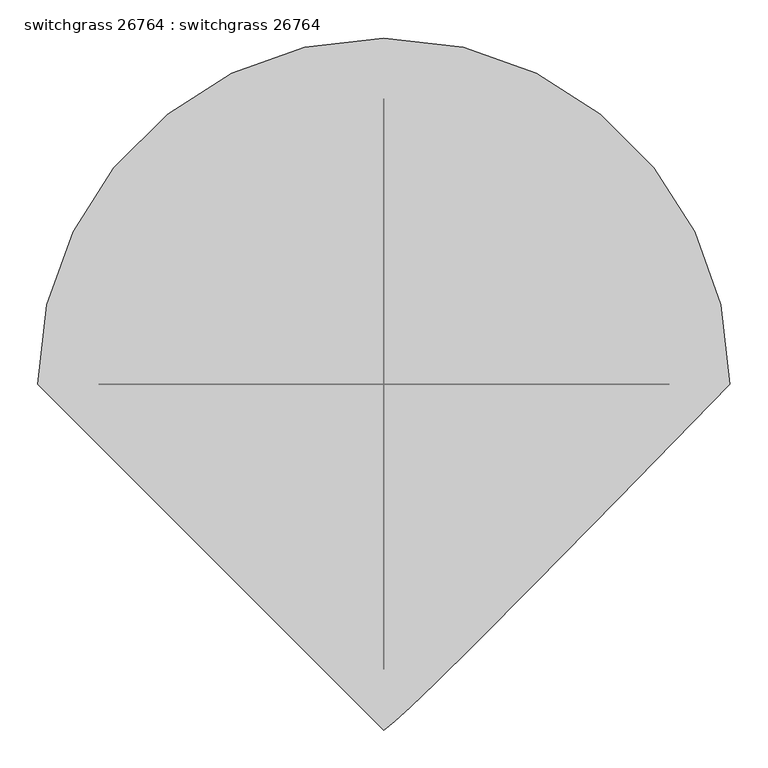
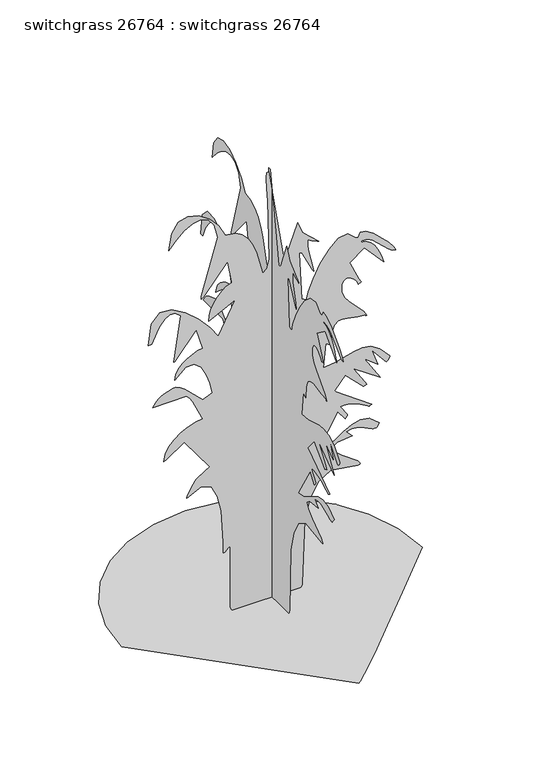
"""IFC4 building model written with IfcOpenShell, lengths in millimetres: proxy geometry, switchgrass 26764 : switchgrass 26764."""

from ifc_helpers import new_model, si_unit, origin, place, context, project, spatial, triangles, source, transform, mapped, element, save


def switchgrass_26764_switchgrass_26764_1a5b5e56(model_context):
    return source(origin(), model_context, "Body", "Tessellation", [
        triangles([(-457.5348269, 0.0, 5.72e-05), (-445.4393443, 104.8366151, 5.72e-05), (-410.9893759, 201.1121793, 5.72e-05), (-356.9483794, 286.0697479, 5.72e-05), (-286.0697479, 356.9483794, 5.72e-05), (-201.1121793, 410.9893759, 5.72e-05), (-104.8366151, 445.4393443, 5.72e-05), (2e-05, 457.5348269, 5.72e-05), (104.8366151, 445.4393443, 5.72e-05), (201.1124336, 410.9893759, 5.72e-05), (286.0697479, 356.9483794, 5.72e-05), (356.9483794, 286.0697479, 5.72e-05), (410.9893759, 201.1121793, 5.72e-05), (445.4393443, 104.8366151, 5.72e-05), (457.5348269, -4e-05, 5.72e-05), (308.8459013, -152.5179615, 5.72e-05), (198.615602, -264.8099809, 5.72e-05), (120.4339824, -343.5803727, 5.72e-05), (67.8913365, -395.5334879, 5.72e-05), (34.5780016, -427.3748946, 5.72e-05), (14.0840831, -445.8076721, 5.72e-05), (-6e-05, -457.5348269, 5.72e-05), (34.93284, -5.5e-06, 1088.4574717), (36.237382, -5.5e-06, 1088.5946726), (37.9539129, -5.5e-06, 1088.9655075), (39.8896437, -5.5e-06, 1089.5065355), (41.8515379, -5.4e-06, 1090.1567139), (43.6465546, -5.4e-06, 1090.8526743), (45.0816551, -5.3e-06, 1091.5334467), (45.9643001, -5.3e-06, 1092.1353722), (79.0584374, -3e-07, 1176.7097157), (93.7670509, -2.4e-06, 1139.9381956), (141.570056, -5.1e-06, 1095.8133453), (139.9581813, -5e-06, 1096.2705122), (120.3097713, -3.5e-06, 1104.9699812), (109.4510318, -2.7e-06, 1111.5257584), (108.7718309, -3.8e-06, 1094.9344746), (110.1157441, -4.9e-06, 1079.5497305), (124.110375, -9.5e-06, 1020.4566805), (126.8614426, -1.06e-05, 1003.8832008), (124.028585, -1.03e-05, 1007.8913137), (90.0899044, -6.2e-06, 1077.4263136), (82.7355931, -6.2e-06, 1077.4263136), (90.0899044, -1.52e-05, 926.664731), (91.5981517, -1.52e-05, 926.3243448), (93.839948, -1.52e-05, 925.4277426), (96.493992, -1.53e-05, 924.1679358), (99.2384648, -1.54e-05, 922.7353924), (101.7517925, -1.55e-05, 921.3205805), (103.7124104, -1.55e-05, 920.1165842), (104.7985178, -1.56e-05, 919.30893), (110.3578079, -1.41e-05, 944.2085003), (125.3806282, -1.19e-05, 981.1629307), (147.3843723, -9.5e-06, 1022.163553), (173.8869515, -7.3e-06, 1059.1942142), (202.4055415, -5.8e-06, 1084.2512604), (230.4577718, -5.5e-06, 1089.3210817), (255.5618354, -6.8e-06, 1066.3950829), (262.9151293, -6.8e-06, 1066.3950829), (269.3514915, -6.1e-06, 1080.2456909), (285.9199024, -6.4e-06, 1077.2713085), (308.5106383, -7.4e-06, 1062.4834757), (355.3227882, -1.03e-05, 1017.5331671), (371.3222114, -1.13e-05, 997.3934807), (376.9076989, -1.17e-05, 985.4987125), (366.3362148, -1.13e-05, 987.6501074), (353.3212752, -1.07e-05, 997.467168), (306.0061764, -8.2e-06, 1041.5234179), (289.6028898, -7.7e-06, 1050.6166128), (273.9463418, -7.7e-06, 1051.6859516), (270.2709666, -7.9e-06, 1048.0105946), (286.0621357, -8.1e-06, 1044.6704641), (300.011793, -8.7e-06, 1035.6788618), (312.0590046, -9.4e-06, 1022.5750105), (322.1529742, -1.04e-05, 1006.8905754), (330.2352207, -1.14e-05, 990.169721), (336.2473901, -1.23e-05, 973.9468014), (340.1361425, -1.32e-05, 959.7583506), (281.3021792, -9.2e-06, 1025.9481331), (237.175821, -1.12e-05, 992.8519701), (237.8959079, -1.14e-05, 989.6693882), (264.7083701, -1.53e-05, 931.0716568), (271.2971213, -1.6e-05, 919.3597263), (262.201401, -1.58e-05, 915.7986065), (257.5227259, -1.51e-05, 925.7833895), (250.3543407, -1.46e-05, 934.7876364), (241.7117542, -1.42e-05, 941.820928), (232.6099115, -1.39e-05, 945.8899384), (224.0638488, -1.4e-05, 946.014422), (217.0887659, -1.43e-05, 941.1985823), (212.6996442, -1.49e-05, 930.4569414), (212.5952538, -1.63e-05, 907.9474869), (220.1395426, -1.74e-05, 888.4809425), (232.934274, -1.85e-05, 871.1581627), (278.8409195, -2.13e-05, 823.0557209), (288.6554731, -2.24e-05, 805.3188675), (284.9775544, -2.24e-05, 805.3188675), (284.9775544, -2.22e-05, 808.9968407), (261.1244319, -2.2e-05, 811.3030952), (219.0793602, -2.16e-05, 819.2355326), (202.3661725, -2.16e-05, 817.8461552), (189.5122514, -2.22e-05, 808.2093887), (181.2572684, -2.35e-05, 786.8149824), (178.341349, -2.57e-05, 750.1603157), (163.6327264, -2.52e-05, 757.5161167), (156.2784152, -2.96e-05, 683.9730766), (191.325313, -2.94e-05, 687.4935013), (248.5903132, -2.85e-05, 703.0763437), (274.1444584, -2.83e-05, 706.7441431), (299.8746466, -2.85e-05, 702.0628881), (327.443785, -2.96e-05, 684.8417009), (358.5206308, -3.16e-05, 650.8794571), (358.1040865, -3.17e-05, 648.5070728), (356.9788645, -3.19e-05, 645.8020054), (355.3380126, -3.21e-05, 643.0156202), (353.374615, -3.22e-05, 640.4019716), (351.2841903, -3.24e-05, 638.2225988), (349.2598226, -3.24e-05, 636.7265419), (347.4894364, -3.25e-05, 636.1703259), (303.3646043, -2.94e-05, 687.6509771), (321.6983145, -3.25e-05, 637.1100941), (281.4164709, -3.05e-05, 668.6899252), (329.1049481, -3.51e-05, 592.0454756), (248.2070336, -3.18e-05, 647.2014839), (249.7422051, -3.2e-05, 643.9071356), (282.1810136, -3.5e-05, 593.8082314), (288.6554731, -3.55e-05, 584.6896382), (287.7740952, -3.56e-05, 584.486453), (278.9298131, -3.57e-05, 581.2174664), (277.6242605, -3.58e-05, 581.0117014), (222.4671985, -3.25e-05, 636.1703259), (189.3728159, -3.49e-05, 595.7208326), (303.3646043, -3.97e-05, 514.8244623), (302.6254598, -3.97e-05, 514.6872977), (301.5739069, -3.97e-05, 514.3164628), (300.3369185, -3.98e-05, 513.7754348), (299.0364347, -3.98e-05, 513.1252201), (297.7994644, -3.98e-05, 512.4292597), (296.7479115, -3.99e-05, 511.7485236), (296.008767, -3.99e-05, 511.1465618), (285.8436898, -3.91e-05, 517.9918562), (258.9959281, -3.82e-05, 530.9178841), (230.2492453, -3.8e-05, 539.6935839), (217.7123288, -3.81e-05, 541.3522036), (207.7585759, -3.82e-05, 540.564788), (229.8212554, -4.01e-05, 507.4711684), (229.5405858, -4.03e-05, 505.7007823), (228.7854538, -4.04e-05, 503.6738711), (227.6866473, -4.05e-05, 501.5834464), (226.3747361, -4.06e-05, 499.6225923), (224.9802718, -4.07e-05, 497.9817404), (223.6343329, -4.08e-05, 496.8565184), (222.4671985, -4.08e-05, 496.4374306), (200.4042828, -3.9e-05, 525.8556567), (137.8929095, -4.54e-05, 419.2189608), (166.0807783, -4.51e-05, 424.9746051), (192.3560459, -4.44e-05, 438.7921846), (217.6356256, -4.35e-05, 455.4799742), (242.8367037, -4.28e-05, 469.858893), (268.8765023, -4.25e-05, 476.7397593), (296.6716989, -4.29e-05, 470.9409127), (327.1389708, -4.44e-05, 447.2757874), (326.9992627, -4.44e-05, 446.6026817), (318.6350567, -4.45e-05, 435.0634515), (318.0737174, -4.45e-05, 433.928092), (304.8454187, -4.44e-05, 435.7644988), (292.8515469, -4.41e-05, 440.3060094), (269.6842292, -4.35e-05, 451.6369311), (257.0629792, -4.32e-05, 455.5028289), (242.7904856, -4.32e-05, 456.2140137), (226.1443541, -4.34e-05, 452.3125803), (244.5298779, -4.45e-05, 433.928092), (198.3082625, -4.53e-05, 429.3560964), (183.5841612, -4.73e-05, 417.3698367), (191.3966749, -5e-05, 400.5525129), (212.7859943, -5.3e-05, 381.4872886), (260.4513443, -5.75e-05, 346.9661762), (268.8053947, -5.81e-05, 336.6766517), (266.5219404, -5.8e-05, 334.0198371), (261.1066641, -5.8e-05, 333.3340141), (178.1579663, -6e-05, 346.4759809), (140.1265758, -6.16e-05, 322.2393062), (114.9013532, -6.35e-05, 274.7464384), (99.9910624, -6.53e-05, 212.9973368), (92.4787665, -7.02e-05, 12.5836557), (91.8127825, -7.03e-05, 8.321819), (90.5290672, -7.04e-05, 4.9722738), (88.4818266, -7.04e-05, 2.3959441), (85.5242583, -7.04e-05, 0.4537325), (-118.3633693, -7.08e-05, 2.4e-05), (-122.0969169, -7.09e-05, 2.3783469), (-124.6485962, -7.1e-05, 5.1976728), (-126.2274606, -7.11e-05, 8.3395482), (-127.0420366, -7.12e-05, 11.6852833), (-127.3018772, -7.12e-05, 15.1165158), (-126.9912402, -7.13e-05, 21.7608447), (-126.8614426, -5.81e-05, 205.9442608), (-129.3712185, -5.82e-05, 207.0623793), (-132.5175108, -5.83e-05, 205.407811), (-143.2413748, -5.85e-05, 195.0563171), (-146.3985949, -5.86e-05, 193.5589884), (-148.9243673, -5.88e-05, 194.9127939), (-148.7935613, -5.68e-05, 227.8207598), (-154.894379, -5.06e-05, 331.9700349), (-165.8895291, -4.76e-05, 382.8233262), (-185.3575813, -4.54e-05, 419.2723005), (-215.6798221, -4.47e-05, 431.1264825), (-259.2397541, -4.61e-05, 408.1877664), (-259.6156759, -4.59e-05, 410.1283092), (-257.8935608, -4.56e-05, 415.3124405), (-244.622078, -4.41e-05, 440.6336783), (-233.4986654, -4.32e-05, 455.9905171), (-232.2906359, -4.31e-05, 458.4568274), (-228.0976142, -4.28e-05, 462.3633476), (-205.3272926, -4.19e-05, 477.5550802), (-189.3728159, -4.15e-05, 485.4061998), (-266.593048, -3.51e-05, 592.0454756), (-321.7491108, -3.73e-05, 555.2739192), (-329.1049481, -3.75e-05, 551.5960187), (-325.1247405, -3.62e-05, 573.5644452), (-314.238341, -3.5e-05, 593.5542134), (-298.0255225, -3.4e-05, 611.0903887), (-278.058609, -3.31e-05, 625.6979273), (-255.9199894, -3.24e-05, 636.9018219), (-233.1864933, -3.2e-05, 644.2271742), (-211.4357316, -3.18e-05, 647.2014839), (-213.7123368, -3.13e-05, 653.8029705), (-240.9860717, -2.74e-05, 712.3753401), (-250.6378082, -2.7e-05, 726.9625311), (-260.7383544, -2.74e-05, 738.2883659), (-362.9504113, -3.12e-05, 737.0260157), (-353.9791203, -3.02e-05, 749.4745291), (-345.6987391, -2.91e-05, 758.1181149), (-337.7028245, -2.78e-05, 763.9169615), (-329.5900566, -2.65e-05, 767.8437567), (-300.461384, -2.23e-05, 778.026638), (-293.1055467, -2.23e-05, 778.026638), (-278.8536186, -2.33e-05, 770.8663919), (-266.2755528, -2.42e-05, 762.6672558), (-211.4357316, -2.81e-05, 709.7133659), (-182.0185046, -2.74e-05, 720.7445967), (-189.8899537, -2.53e-05, 755.5907982), (-200.3534683, -2.34e-05, 786.4390606), (-215.7232605, -2.17e-05, 814.9480036), (-236.4161108, -2.06e-05, 832.6416183), (-262.8490904, -2.07e-05, 831.0515991), (-295.4347286, -2.24e-05, 801.707024), (-292.5975471, -2.14e-05, 818.2246204), (-284.8327776, -2.06e-05, 832.9972652), (-273.265624, -1.99e-05, 845.8724968), (-259.0162394, -1.93e-05, 856.6852816), (-243.2146603, -1.88e-05, 865.2806145), (-226.9795139, -1.84e-05, 871.5010923), (-211.4357316, -1.82e-05, 875.1840797), (-229.8215097, -1.43e-05, 941.3738623), (-296.0113104, -1.91e-05, 860.4749485), (-299.6866857, -1.91e-05, 860.4749485), (-277.7029984, -1e-05, 1003.3269121), (-294.71337, -9.2e-06, 1017.2435772), (-311.0531794, -9.3e-06, 1017.8481188), (-326.2398251, -9.9e-06, 1008.5745569), (-339.7957927, -1.1e-05, 992.857057), (-351.2410243, -1.22e-05, 974.1270956), (-365.8764682, -1.43e-05, 941.3738623), (-376.9076989, -1.43e-05, 941.3738623), (-367.2226796, -1.04e-05, 1007.1064779), (-341.7211112, -8.7e-06, 1034.375889), (-305.7369704, -8.9e-06, 1031.8511158), (-264.604234, -1.03e-05, 1008.203722), (-223.6538811, -1.25e-05, 972.1078148), (-188.2191436, -1.48e-05, 932.229871), (-163.6329808, -1.69e-05, 897.2464685), (-112.1528291, -1.1e-05, 996.5298706), (-193.0499715, -1.34e-05, 956.0804501), (-191.1398955, -1.24e-05, 973.1822405), (-185.7319771, -1.13e-05, 990.7996971), (-177.3111248, -1.03e-05, 1008.0386158), (-166.3611936, -9.4e-06, 1024.0076265), (-153.3675827, -8.5e-06, 1037.8124525), (-138.8136563, -7.9e-06, 1048.5617237), (-123.1842869, -7.5e-06, 1055.3638521), (-122.7161651, -7.3e-06, 1058.0105656), (-134.2157538, -3.3e-06, 1125.2290644), (-138.2424067, -3.4e-06, 1124.548292), (-207.9053874, -8.4e-06, 1039.524412), (-215.1128872, -8.8e-06, 1033.3014633), (-214.9937629, -6.5e-06, 1043.3674913), (-165.5864953, 2.1e-06, 1216.2397156), (-176.4513299, 4.6e-06, 1258.3223213), (-194.0382833, 6.1e-06, 1282.2669353), (-216.3737477, 6.6e-06, 1290.7911243), (-241.4831526, 6.4e-06, 1286.6001011), (-267.3931445, 5.6e-06, 1272.4143391), (-292.1276449, 4.3e-06, 1250.938615), (-313.7150808, 2.8e-06, 1224.8909317), (-305.8919028, 5.9e-06, 1277.1868675), (-285.2950496, 7.5e-06, 1305.4849949), (-256.2374846, 8e-06, 1313.3996281), (-223.0242321, 7.4e-06, 1304.5427559), (-189.9694546, 6.1e-06, 1282.5285473), (-161.3812832, 4.2e-06, 1250.9716072), (-141.570056, 1.9e-06, 1213.4812357), (-111.003735, 1.7e-06, 1210.2630455), (-90.0827918, 1e-06, 1197.192259), (-72.9868286, -2e-07, 1178.0406664), (-59.2218167, -1.6e-06, 1154.5431181), (-48.2927191, -3.1e-06, 1128.4294504), (-27.578531, -7.7e-06, 1051.6859516), (-15.6259369, -7e-06, 1062.9330849), (-8.9939533, -5.3e-06, 1092.3284563), (-12.8700152, 6.1e-06, 1283.3463753), (-14.1246216, 5.9e-06, 1292.5767712), (-15.1875847, 6.3e-06, 1303.493692), (-16.0281459, 7e-06, 1315.7644547), (-16.6151389, 8.1e-06, 1329.0460567), (-16.9180092, 9.2e-06, 1343.0058151), (-16.9057404, 1.04e-05, 1357.3034889), (-16.5471686, 1.14e-05, 1371.5986919), (-9.1928857, 1.14e-05, 1371.5986919), (-3.16e-05, -34.93284, 1088.4574717), (-3.16e-05, -36.237382, 1088.5946726), (-3.16e-05, -37.9539129, 1088.9655075), (-3.16e-05, -39.8896437, 1089.509079), (-3.16e-05, -41.8515379, 1090.1567139), (-3.16e-05, -43.6465546, 1090.8552177), (-3.16e-05, -45.0819049, 1091.5334467), (-3.16e-05, -45.9643001, 1092.1353722), (-3.16e-05, -79.0586918, 1176.7097157), (-3.16e-05, -93.7673053, 1139.9381956), (-3.16e-05, -141.570056, 1095.8133453), (-3.15e-05, -139.9581813, 1096.2705122), (-3.05e-05, -120.3097713, 1104.9699812), (-3.01e-05, -109.4512861, 1111.5257584), (-3.02e-05, -108.7720852, 1094.9344746), (-3.04e-05, -110.1157441, 1079.5497305), (-3.15e-05, -124.1106294, 1020.4566805), (-3.16e-05, -126.8614426, 1003.8832008), (-3.16e-05, -124.028585, 1007.8913137), (-3.16e-05, -90.0901496, 1077.4263136), (-3.16e-05, -82.7358474, 1077.4263136), (-3.16e-05, -90.0901496, 926.664731), (-3.16e-05, -91.5981517, 926.3243448), (-3.16e-05, -93.8402023, 925.4277426), (-3.16e-05, -96.493992, 924.1679358), (-3.16e-05, -99.2387191, 922.7353924), (-3.16e-05, -101.7517925, 921.3205805), (-3.16e-05, -103.7124104, 920.1165842), (-3.16e-05, -104.7985178, 919.30893), (-3.16e-05, -110.3578079, 944.2085003), (-3.16e-05, -125.3806282, 981.1629307), (-3.16e-05, -147.3846266, 1022.163553), (-3.16e-05, -173.8872059, 1059.1942142), (-3.16e-05, -202.4055415, 1084.2512604), (-3.16e-05, -230.4580261, 1089.3210817), (-3.16e-05, -255.5618354, 1066.3950829), (-3.16e-05, -262.9151293, 1066.3950829), (-3.16e-05, -269.3514915, 1080.2456909), (-3.18e-05, -285.9199024, 1077.2713085), (-3.19e-05, -308.5106383, 1062.4834757), (-3.21e-05, -355.3227882, 1017.5331671), (-3.19e-05, -371.3222114, 997.3934807), (-3.16e-05, -376.9076989, 985.4987125), (-3.14e-05, -366.3362148, 987.6501074), (-3.13e-05, -353.3212752, 997.467168), (-3.14e-05, -306.0061764, 1041.5234179), (-3.15e-05, -289.6028898, 1050.6166128), (-3.16e-05, -273.9463418, 1051.6859516), (-3.16e-05, -270.2709666, 1048.0105946), (-3.16e-05, -286.0621357, 1044.6704641), (-3.16e-05, -300.011793, 1035.6788618), (-3.16e-05, -312.0590046, 1022.5750105), (-3.16e-05, -322.1529742, 1006.8905754), (-3.16e-05, -330.2352207, 990.169721), (-3.16e-05, -336.2473901, 973.9468014), (-3.16e-05, -340.1361425, 959.7583506), (-3.16e-05, -281.3021792, 1025.9481331), (-3.16e-05, -237.175821, 992.8519701), (-3.16e-05, -237.8959079, 989.6693882), (-3.19e-05, -264.7083701, 931.0716568), (-3.19e-05, -271.2971213, 919.3597263), (-3.16e-05, -262.201401, 915.7986065), (-3.15e-05, -257.5227259, 925.7833895), (-3.15e-05, -250.3543407, 934.7876364), (-3.15e-05, -241.7117542, 941.820928), (-3.15e-05, -232.6099115, 945.8924818), (-3.15e-05, -224.0641032, 946.014422), (-3.15e-05, -217.0887659, 941.1985823), (-3.16e-05, -212.6996442, 930.4569414), (-3.16e-05, -212.5955081, 907.9474869), (-3.16e-05, -220.1397969, 888.4809425), (-3.16e-05, -232.934274, 871.1581627), (-3.16e-05, -278.8409195, 823.0557209), (-3.16e-05, -288.6554731, 805.3188675), (-3.16e-05, -284.9775544, 805.3188675), (-3.16e-05, -284.9775544, 808.9968407), (-3.16e-05, -261.1244319, 811.3030952), (-3.16e-05, -219.0796145, 819.2355326), (-3.16e-05, -202.3661725, 817.8461552), (-3.16e-05, -189.5122514, 808.2093887), (-3.16e-05, -181.2575227, 786.8149824), (-3.16e-05, -178.3416033, 750.1603157), (-3.16e-05, -163.6329808, 757.5161167), (-3.16e-05, -156.2786695, 683.9730766), (-3.16e-05, -191.325313, 687.4935013), (-3.16e-05, -248.5905676, 703.0763437), (-3.16e-05, -274.1444584, 706.7441431), (-3.16e-05, -299.8746466, 702.0628881), (-3.16e-05, -327.443785, 684.8417009), (-3.16e-05, -358.5206308, 650.8794571), (-3.16e-05, -358.1040865, 648.5070728), (-3.16e-05, -356.9788645, 645.8020054), (-3.16e-05, -355.3380126, 643.0156202), (-3.16e-05, -353.374615, 640.4019716), (-3.16e-05, -351.2841903, 638.2225988), (-3.16e-05, -349.2598226, 636.7265419), (-3.16e-05, -347.4894364, 636.1703259), (-3.16e-05, -303.3646043, 687.6509771), (-3.17e-05, -321.6983145, 637.1100941), (-3.16e-05, -281.4164709, 668.6899252), (-3.16e-05, -329.1049481, 592.0454756), (-3.16e-05, -248.2072879, 647.2014839), (-3.16e-05, -249.7422051, 643.9071356), (-3.16e-05, -282.1810136, 593.8082314), (-3.16e-05, -288.6554731, 584.6896382), (-3.16e-05, -287.7740952, 584.486453), (-3.16e-05, -278.9298131, 581.2174664), (-3.16e-05, -277.6242605, 581.0117014), (-3.16e-05, -222.4671985, 636.1703259), (-3.16e-05, -189.3728159, 595.7208326), (-3.16e-05, -303.3646043, 514.8244623), (-3.16e-05, -302.6254598, 514.6872977), (-3.16e-05, -301.5739069, 514.3164628), (-3.16e-05, -300.3369185, 513.7754348), (-3.16e-05, -299.0364347, 513.1252201), (-3.16e-05, -297.7994644, 512.4292597), (-3.16e-05, -296.7479115, 511.7485236), (-3.16e-05, -296.0113104, 511.1465618), (-3.12e-05, -285.8436898, 517.9918562), (-3.1e-05, -258.9959281, 530.9178841), (-3.13e-05, -230.2494996, 539.6935839), (-3.15e-05, -217.7125832, 541.3522036), (-3.16e-05, -207.7585759, 540.564788), (-3.16e-05, -229.8215097, 507.4711684), (-3.16e-05, -229.5408401, 505.7007823), (-3.16e-05, -228.7857081, 503.6738711), (-3.16e-05, -227.6866473, 501.5834464), (-3.16e-05, -226.3747361, 499.6225923), (-3.16e-05, -224.9805262, 497.9817404), (-3.16e-05, -223.6343329, 496.8565184), (-3.16e-05, -222.4671985, 496.4374306), (-3.16e-05, -200.4042828, 525.8556567), (-3.16e-05, -137.8929095, 419.2189608), (-3.16e-05, -166.0807783, 424.9771485), (-3.17e-05, -192.3560459, 438.7921846), (-3.18e-05, -217.63588, 455.4799742), (-3.19e-05, -242.8367037, 469.858893), (-3.21e-05, -268.8765023, 476.7397593), (-3.21e-05, -296.6716989, 470.9409127), (-3.22e-05, -327.1389708, 447.2757874), (-3.21e-05, -326.9992627, 446.6026817), (-3.16e-05, -318.6350567, 435.0634515), (-3.16e-05, -318.0737174, 433.928092), (-3.16e-05, -304.8454187, 435.7644988), (-3.16e-05, -292.8540904, 440.3060094), (-3.16e-05, -269.6842292, 451.6369311), (-3.16e-05, -257.0629792, 455.5028289), (-3.16e-05, -242.7904856, 456.2140137), (-3.16e-05, -226.1443541, 452.3125803), (-3.16e-05, -244.5301323, 433.928092), (-3.21e-05, -198.3082625, 429.3560964), (-3.33e-05, -183.5841612, 417.3698367), (-3.51e-05, -191.3969293, 400.5525129), (-3.69e-05, -212.7862487, 381.4872886), (-3.94e-05, -260.4513443, 346.9661762), (-3.94e-05, -268.8053947, 336.6766517), (-3.91e-05, -266.5219404, 334.0198371), (-3.91e-05, -261.1066641, 333.3340141), (-4.18e-05, -178.1579663, 346.4759809), (-4.2e-05, -140.1265758, 322.2393062), (-4.1e-05, -114.9013532, 274.7464384), (-3.92e-05, -99.9910624, 212.9973368), (-3.21e-05, -92.4787665, 12.5836296), (-3.2e-05, -91.8127825, 8.3217934), (-3.19e-05, -90.5293216, 4.9722483), (-3.18e-05, -88.4818266, 2.3959185), (-3.16e-05, -85.5242583, 0.4537071), (-3.19e-05, 118.3631241, 0.0), (-3.22e-05, 122.0966625, 2.378324), (-3.24e-05, 124.6483418, 5.1976479), (-3.27e-05, 126.2272062, 8.3395226), (-3.3e-05, 127.0420366, 11.6852833), (-3.33e-05, 127.3018772, 15.1164896), (-3.38e-05, 126.9912402, 21.7608197), (-3.16e-05, 126.8614426, 205.9442608), (-3.17e-05, 129.3709642, 207.062125), (-3.17e-05, 132.5175108, 205.407811), (-3.13e-05, 143.2413748, 195.0563171), (-3.13e-05, 146.3985949, 193.5589884), (-3.16e-05, 148.924113, 194.9127939), (-3.16e-05, 148.7935613, 227.8207598), (-3.16e-05, 154.8941247, 331.9700349), (-3.16e-05, 165.8895291, 382.8233262), (-3.16e-05, 185.357327, 419.274844), (-3.16e-05, 215.6798221, 431.1264825), (-3.16e-05, 259.2397541, 408.1877664), (-3.16e-05, 259.6156759, 410.1283092), (-3.16e-05, 257.8935608, 415.3124405), (-3.16e-05, 244.6218236, 440.6336783), (-3.16e-05, 233.498411, 455.9905171), (-3.16e-05, 232.2906359, 458.4568274), (-3.16e-05, 228.0976142, 462.3658911), (-3.16e-05, 205.3272926, 477.5550802), (-3.16e-05, 189.3728159, 485.4061998), (-3.16e-05, 266.593048, 592.0454756), (-3.16e-05, 321.7491108, 555.2739192), (-3.16e-05, 329.1049481, 551.5960187), (-3.16e-05, 325.1247405, 573.5644452), (-3.16e-05, 314.238341, 593.5542134), (-3.16e-05, 298.0229791, 611.0903887), (-3.16e-05, 278.058609, 625.6979273), (-3.16e-05, 255.9199894, 636.9018219), (-3.16e-05, 233.186239, 644.2271742), (-3.16e-05, 211.4357316, 647.2014839), (-3.14e-05, 213.7123368, 653.8029705), (-3.1e-05, 240.9858174, 712.3753401), (-3.15e-05, 250.6378082, 726.9625311), (-3.26e-05, 260.7383544, 738.2883659), (-3.63e-05, 362.9504113, 737.0260157), (-3.61e-05, 353.9765768, 749.4745291), (-3.54e-05, 345.6987391, 758.1181149), (-3.45e-05, 337.7028245, 763.9169615), (-3.34e-05, 329.5900566, 767.8437567), (-2.99e-05, 300.461384, 778.026638), (-2.99e-05, 293.1055467, 778.026638), (-3.04e-05, 278.8536186, 770.8663919), (-3.08e-05, 266.2730093, 762.6672558), (-3.16e-05, 211.4357316, 709.7133659), (-3.16e-05, 182.0185046, 720.7445967), (-3.15e-05, 189.8899537, 755.5907982), (-3.15e-05, 200.353214, 786.4390606), (-3.15e-05, 215.7232605, 814.9480036), (-3.14e-05, 236.4161108, 832.6416183), (-3.14e-05, 262.8465652, 831.0515991), (-3.14e-05, 295.4347286, 801.707024), (-3.14e-05, 292.5975471, 818.2246204), (-3.14e-05, 284.8327776, 832.9972652), (-3.15e-05, 273.265624, 845.8724968), (-3.15e-05, 259.0162394, 856.6852816), (-3.15e-05, 243.2146603, 865.2806145), (-3.16e-05, 226.9795139, 871.5010923), (-3.16e-05, 211.4357316, 875.1840797), (-3.16e-05, 229.8212554, 941.3738623), (-3.16e-05, 296.008767, 860.4749485), (-3.16e-05, 299.6866857, 860.4749485), (-3.1e-05, 277.7029984, 1003.3269121), (-3.1e-05, 294.71337, 1017.2435772), (-3.11e-05, 311.0531794, 1017.8481188), (-3.12e-05, 326.2398251, 1008.5745569), (-3.13e-05, 339.7957927, 992.857057), (-3.14e-05, 351.2384809, 974.1270956), (-3.16e-05, 365.8764682, 941.3738623), (-3.16e-05, 376.9076989, 941.3738623), (-3.16e-05, 367.2226796, 1007.1064779), (-3.16e-05, 341.7211112, 1034.375889), (-3.16e-05, 305.7369704, 1031.8511158), (-3.16e-05, 264.604234, 1008.203722), (-3.16e-05, 223.6538811, 972.1078148), (-3.16e-05, 188.2191436, 932.229871), (-3.16e-05, 163.6327264, 897.2464685), (-3.16e-05, 112.1528291, 996.5298706), (-3.16e-05, 193.0499715, 956.0804501), (-3.16e-05, 191.1396412, 973.1822405), (-3.16e-05, 185.7317227, 990.7996971), (-3.16e-05, 177.3108705, 1008.0386158), (-3.16e-05, 166.3611936, 1024.0076265), (-3.16e-05, 153.3673283, 1037.8124525), (-3.16e-05, 138.813402, 1048.5617237), (-3.16e-05, 123.1842869, 1055.3638521), (-3.16e-05, 122.7159107, 1058.0105656), (-3.16e-05, 134.2157538, 1125.2290644), (-3.16e-05, 138.2424067, 1124.548292), (-3.16e-05, 207.9053874, 1039.524412), (-3.16e-05, 215.1128872, 1033.3014633), (-2.99e-05, 214.9935086, 1043.3674913), (-3.16e-05, 165.5864953, 1216.2397156), (-3.16e-05, 176.4510756, 1258.3223213), (-3.15e-05, 194.0382833, 1282.2669353), (-3.15e-05, 216.3737477, 1290.7911243), (-3.15e-05, 241.4828982, 1286.6001011), (-3.14e-05, 267.3931445, 1272.4143391), (-3.14e-05, 292.1276449, 1250.938615), (-3.14e-05, 313.7150808, 1224.8909317), (-3.14e-05, 305.8919028, 1277.1868675), (-3.14e-05, 285.2950496, 1305.4849949), (-3.15e-05, 256.2349411, 1313.3996281), (-3.15e-05, 223.0242321, 1304.5427559), (-3.15e-05, 189.9694546, 1282.5285473), (-3.16e-05, 161.3812832, 1250.9716072), (-3.16e-05, 141.570056, 1213.4812357), (-3.16e-05, 111.003735, 1210.2630455), (-3.16e-05, 90.0825374, 1197.192259), (-3.16e-05, 72.9865742, 1178.0432098), (-3.16e-05, 59.2215669, 1154.5431181), (-3.16e-05, 48.2927191, 1128.4294504), (-3.16e-05, 27.578531, 1051.6859516), (-3.16e-05, 15.6258108, 1062.9330849), (-3.16e-05, 8.9938517, 1092.3284563), (-3.16e-05, 12.869888, 1283.3463753), (-3.23e-05, 14.1245194, 1292.5767712), (-3.26e-05, 15.1874576, 1303.493692), (-3.26e-05, 16.0280449, 1315.7644547), (-3.23e-05, 16.6150378, 1329.0460567), (-3.2e-05, 16.917907, 1343.0058151), (-3.17e-05, 16.9056394, 1357.3034889), (-3.16e-05, 16.5470675, 1371.5986919), (-3.16e-05, 9.1927591, 1371.5986919)], [[22, 21, 1], [21, 20, 1], [20, 19, 1], [19, 18, 1], [18, 17, 1], [1, 17, 2], [2, 17, 3], [3, 17, 4], [17, 16, 4], [4, 16, 5], [5, 16, 6], [6, 16, 7], [7, 16, 8], [8, 16, 9], [9, 16, 10], [10, 16, 11], [11, 16, 12], [16, 15, 12], [15, 14, 12], [14, 13, 12], [123, 122, 124], [40, 39, 41], [78, 77, 79], [77, 76, 79], [33, 32, 34], [34, 32, 35], [35, 32, 36], [76, 75, 79], [295, 294, 296], [121, 120, 122], [75, 74, 79], [247, 246, 248], [248, 246, 249], [74, 73, 79], [31, 30, 32], [133, 132, 134], [286, 285, 287], [172, 171, 173], [249, 246, 250], [219, 218, 220], [65, 64, 66], [231, 230, 232], [232, 230, 233], [233, 230, 234], [234, 230, 235], [134, 132, 135], [235, 230, 236], [236, 230, 237], [237, 230, 238], [238, 230, 239], [274, 273, 275], [275, 273, 276], [276, 273, 277], [135, 132, 136], [73, 72, 79], [136, 132, 137], [277, 273, 278], [137, 132, 138], [218, 217, 220], [220, 217, 221], [221, 217, 222], [222, 217, 223], [127, 126, 128], [104, 103, 105], [230, 229, 239], [239, 229, 240], [138, 132, 139], [208, 207, 209], [209, 207, 210], [210, 207, 211], [278, 273, 279], [32, 30, 36], [36, 30, 37], [229, 228, 240], [294, 293, 296], [296, 293, 297], [297, 293, 298], [293, 292, 298], [298, 292, 299], [292, 291, 299], [299, 291, 300], [291, 290, 300], [290, 289, 300], [300, 289, 301], [289, 288, 301], [301, 288, 302], [139, 132, 140], [140, 132, 141], [141, 132, 142], [142, 132, 143], [143, 132, 144], [144, 132, 145], [66, 64, 67], [64, 63, 67], [257, 256, 258], [256, 255, 258], [279, 273, 280], [265, 264, 266], [264, 263, 266], [263, 262, 266], [266, 262, 267], [262, 261, 267], [267, 261, 268], [261, 260, 268], [260, 259, 268], [268, 259, 269], [259, 258, 269], [258, 255, 269], [269, 255, 270], [270, 255, 271], [255, 254, 271], [271, 254, 272], [83, 82, 84], [84, 82, 85], [280, 273, 281], [72, 71, 79], [67, 63, 68], [63, 62, 68], [68, 62, 69], [62, 61, 69], [69, 61, 70], [61, 60, 70], [60, 59, 70], [211, 207, 212], [97, 96, 98], [96, 95, 98], [98, 95, 99], [318, 317, 319], [319, 317, 23], [317, 316, 23], [316, 315, 23], [315, 314, 23], [314, 313, 23], [313, 312, 23], [312, 311, 23], [311, 310, 23], [250, 246, 251], [246, 245, 251], [251, 245, 252], [85, 82, 86], [86, 82, 87], [82, 81, 87], [37, 30, 38], [99, 95, 100], [41, 39, 42], [39, 38, 42], [38, 30, 42], [42, 30, 43], [87, 81, 88], [95, 94, 100], [310, 309, 23], [228, 227, 240], [223, 217, 224], [70, 59, 71], [252, 245, 253], [178, 177, 179], [179, 177, 180], [180, 177, 181], [177, 176, 181], [176, 175, 181], [79, 71, 80], [285, 284, 287], [287, 284, 288], [288, 284, 302], [302, 284, 303], [284, 283, 303], [303, 283, 304], [304, 283, 305], [305, 283, 306], [306, 283, 307], [283, 282, 307], [307, 282, 308], [282, 281, 308], [281, 273, 308], [153, 152, 154], [152, 151, 154], [151, 150, 154], [150, 149, 154], [149, 148, 154], [148, 147, 154], [147, 146, 154], [146, 145, 154], [165, 164, 166], [100, 94, 101], [59, 58, 71], [71, 58, 80], [119, 118, 120], [118, 117, 120], [117, 116, 120], [116, 115, 120], [115, 114, 120], [114, 113, 120], [113, 112, 120], [112, 111, 120], [111, 110, 120], [94, 93, 101], [110, 109, 120], [120, 109, 122], [109, 108, 122], [122, 108, 124], [108, 107, 124], [128, 126, 129], [129, 126, 130], [126, 125, 130], [130, 125, 131], [125, 124, 131], [124, 107, 131], [131, 107, 132], [107, 106, 132], [43, 30, 44], [30, 29, 44], [29, 28, 44], [28, 27, 44], [27, 26, 44], [26, 25, 44], [25, 24, 44], [24, 23, 44], [23, 309, 44], [309, 308, 44], [308, 273, 44], [273, 272, 44], [162, 161, 163], [163, 161, 164], [164, 161, 166], [166, 161, 167], [161, 160, 167], [167, 160, 168], [168, 160, 169], [160, 159, 169], [169, 159, 170], [159, 158, 170], [170, 158, 171], [171, 158, 173], [158, 157, 173], [157, 156, 173], [173, 156, 174], [88, 81, 89], [245, 244, 253], [253, 244, 254], [202, 201, 203], [201, 200, 203], [200, 199, 203], [199, 198, 203], [212, 207, 213], [213, 207, 214], [207, 206, 214], [214, 206, 215], [215, 206, 216], [58, 57, 80], [57, 56, 80], [56, 55, 80], [55, 54, 80], [54, 53, 80], [80, 53, 81], [81, 53, 89], [89, 53, 90], [53, 52, 90], [90, 52, 91], [52, 51, 91], [91, 51, 92], [92, 51, 93], [93, 51, 101], [101, 51, 102], [254, 244, 272], [244, 243, 272], [272, 243, 44], [243, 242, 44], [242, 241, 44], [224, 217, 225], [217, 216, 225], [225, 216, 226], [102, 51, 103], [103, 51, 105], [44, 241, 45], [45, 241, 46], [46, 241, 47], [47, 241, 48], [48, 241, 49], [49, 241, 50], [50, 241, 51], [51, 241, 105], [105, 241, 106], [106, 241, 132], [132, 241, 145], [145, 241, 154], [154, 241, 155], [241, 240, 155], [240, 227, 155], [227, 226, 155], [226, 216, 155], [216, 206, 155], [206, 205, 155], [205, 204, 155], [204, 203, 155], [203, 198, 155], [198, 197, 155], [181, 175, 182], [175, 174, 182], [174, 156, 182], [156, 155, 182], [155, 197, 182], [182, 197, 183], [183, 197, 184], [197, 196, 184], [184, 196, 185], [185, 196, 186], [186, 196, 187], [187, 196, 188], [188, 196, 189], [189, 196, 190], [196, 195, 190], [195, 194, 190], [190, 194, 191], [191, 194, 192], [192, 194, 193], [420, 419, 421], [337, 336, 338], [375, 374, 376], [374, 373, 376], [330, 329, 331], [331, 329, 332], [332, 329, 333], [373, 372, 376], [592, 591, 593], [418, 417, 419], [372, 371, 376], [544, 543, 545], [545, 543, 546], [371, 370, 376], [328, 327, 329], [430, 429, 431], [583, 582, 584], [469, 468, 470], [546, 543, 547], [516, 515, 517], [362, 361, 363], [528, 527, 529], [529, 527, 530], [530, 527, 531], [531, 527, 532], [431, 429, 432], [532, 527, 533], [533, 527, 534], [534, 527, 535], [535, 527, 536], [571, 570, 572], [572, 570, 573], [573, 570, 574], [432, 429, 433], [370, 369, 376], [433, 429, 434], [574, 570, 575], [434, 429, 435], [515, 514, 517], [517, 514, 518], [518, 514, 519], [519, 514, 520], [424, 423, 425], [401, 400, 402], [527, 526, 536], [536, 526, 537], [435, 429, 436], [505, 504, 506], [506, 504, 507], [507, 504, 508], [575, 570, 576], [329, 327, 333], [333, 327, 334], [526, 525, 537], [591, 590, 593], [593, 590, 594], [594, 590, 595], [590, 589, 595], [595, 589, 596], [589, 588, 596], [596, 588, 597], [588, 587, 597], [587, 586, 597], [597, 586, 598], [586, 585, 598], [598, 585, 599], [436, 429, 437], [437, 429, 438], [438, 429, 439], [439, 429, 440], [440, 429, 441], [441, 429, 442], [363, 361, 364], [361, 360, 364], [554, 553, 555], [553, 552, 555], [576, 570, 577], [562, 561, 563], [561, 560, 563], [560, 559, 563], [563, 559, 564], [559, 558, 564], [564, 558, 565], [558, 557, 565], [557, 556, 565], [565, 556, 566], [556, 555, 566], [555, 552, 566], [566, 552, 567], [567, 552, 568], [552, 551, 568], [568, 551, 569], [380, 379, 381], [381, 379, 382], [577, 570, 578], [369, 368, 376], [364, 360, 365], [360, 359, 365], [365, 359, 366], [359, 358, 366], [366, 358, 367], [358, 357, 367], [357, 356, 367], [508, 504, 509], [394, 393, 395], [393, 392, 395], [395, 392, 396], [615, 614, 616], [616, 614, 320], [614, 613, 320], [613, 612, 320], [612, 611, 320], [611, 610, 320], [610, 609, 320], [609, 608, 320], [608, 607, 320], [547, 543, 548], [543, 542, 548], [548, 542, 549], [382, 379, 383], [383, 379, 384], [379, 378, 384], [334, 327, 335], [396, 392, 397], [338, 336, 339], [336, 335, 339], [335, 327, 339], [339, 327, 340], [384, 378, 385], [392, 391, 397], [607, 606, 320], [525, 524, 537], [520, 514, 521], [367, 356, 368], [549, 542, 550], [475, 474, 476], [476, 474, 477], [477, 474, 478], [474, 473, 478], [473, 472, 478], [376, 368, 377], [582, 581, 584], [584, 581, 585], [585, 581, 599], [599, 581, 600], [581, 580, 600], [600, 580, 601], [601, 580, 602], [602, 580, 603], [603, 580, 604], [580, 579, 604], [604, 579, 605], [579, 578, 605], [578, 570, 605], [450, 449, 451], [449, 448, 451], [448, 447, 451], [447, 446, 451], [446, 445, 451], [445, 444, 451], [444, 443, 451], [443, 442, 451], [462, 461, 463], [397, 391, 398], [356, 355, 368], [368, 355, 377], [416, 415, 417], [415, 414, 417], [414, 413, 417], [413, 412, 417], [412, 411, 417], [411, 410, 417], [410, 409, 417], [409, 408, 417], [408, 407, 417], [391, 390, 398], [407, 406, 417], [417, 406, 419], [406, 405, 419], [419, 405, 421], [405, 404, 421], [425, 423, 426], [426, 423, 427], [423, 422, 427], [427, 422, 428], [422, 421, 428], [421, 404, 428], [428, 404, 429], [404, 403, 429], [340, 327, 341], [327, 326, 341], [326, 325, 341], [325, 324, 341], [324, 323, 341], [323, 322, 341], [322, 321, 341], [321, 320, 341], [320, 606, 341], [606, 605, 341], [605, 570, 341], [570, 569, 341], [459, 458, 460], [460, 458, 461], [461, 458, 463], [463, 458, 464], [458, 457, 464], [464, 457, 465], [465, 457, 466], [457, 456, 466], [466, 456, 467], [456, 455, 467], [467, 455, 468], [468, 455, 470], [455, 454, 470], [454, 453, 470], [470, 453, 471], [385, 378, 386], [542, 541, 550], [550, 541, 551], [499, 498, 500], [498, 497, 500], [497, 496, 500], [496, 495, 500], [509, 504, 510], [510, 504, 511], [504, 503, 511], [511, 503, 512], [512, 503, 513], [355, 354, 377], [354, 353, 377], [353, 352, 377], [352, 351, 377], [351, 350, 377], [377, 350, 378], [378, 350, 386], [386, 350, 387], [350, 349, 387], [387, 349, 388], [349, 348, 388], [388, 348, 389], [389, 348, 390], [390, 348, 398], [398, 348, 399], [551, 541, 569], [541, 540, 569], [569, 540, 341], [540, 539, 341], [539, 538, 341], [521, 514, 522], [514, 513, 522], [522, 513, 523], [399, 348, 400], [400, 348, 402], [341, 538, 342], [342, 538, 343], [343, 538, 344], [344, 538, 345], [345, 538, 346], [346, 538, 347], [347, 538, 348], [348, 538, 402], [402, 538, 403], [403, 538, 429], [429, 538, 442], [442, 538, 451], [451, 538, 452], [538, 537, 452], [537, 524, 452], [524, 523, 452], [523, 513, 452], [513, 503, 452], [503, 502, 452], [502, 501, 452], [501, 500, 452], [500, 495, 452], [495, 494, 452], [478, 472, 479], [472, 471, 479], [471, 453, 479], [453, 452, 479], [452, 494, 479], [479, 494, 480], [480, 494, 481], [494, 493, 481], [481, 493, 482], [482, 493, 483], [483, 493, 484], [484, 493, 485], [485, 493, 486], [486, 493, 487], [493, 492, 487], [492, 491, 487], [487, 491, 488], [488, 491, 489], [489, 491, 490]], closed=False),
    ])


if __name__ == "__main__":
    model = new_model("IFC4")
    model_context = context("Model", 3, world=origin())
    ifc_project = project(units=[si_unit("LENGTHUNIT", "METRE", prefix="MILLI")], contexts=[model_context])
    site = spatial("IfcSite", under=ifc_project)
    building = spatial("IfcBuilding", under=site)
    placement = place(None, origin())
    switchgrass_26764_switchgrass_26764_shape = switchgrass_26764_switchgrass_26764_1a5b5e56(model_context)
    element("IfcBuildingElementProxy", 1, Name="switchgrass 26764 : switchgrass 26764", ObjectType="switchgrass 26764 : switchgrass 26764", at=placement, inside=building, context=model_context, shape_type="MappedRepresentation", body=[
        mapped(switchgrass_26764_switchgrass_26764_shape, transform((0.0, 0.0, 0.0), x_axis=(1.0, 0.0, 0.0), y_axis=(0.0, 1.0, 0.0), z_axis=(0.0, 0.0, 1.0))),
    ])
    save(model, "model.ifc")

# Revit data of these elements
# Type "switchgrass 26764 : switchgrass 26764"
#   built-in parameter 1005195 = "RPC-16-FU2N-0J7X-A2JP-J000-ST1L-LVER-AU"
#   Height = 0
